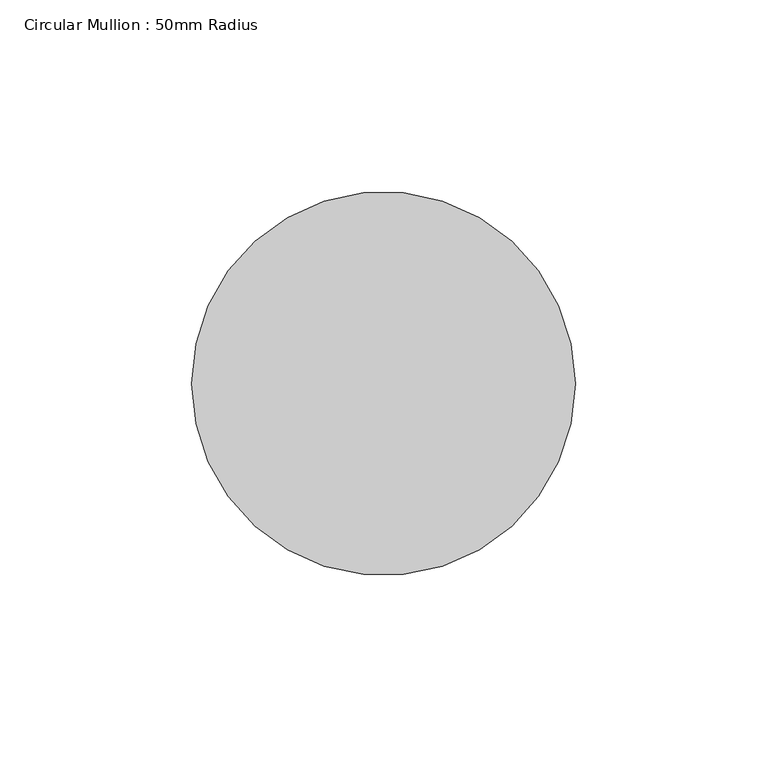
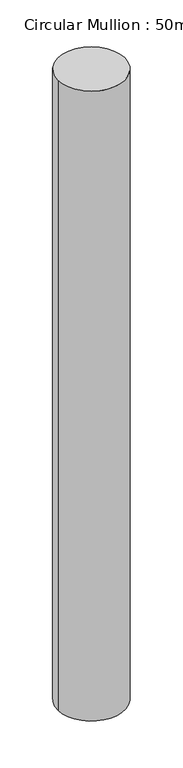
"""IFC4 building model written with IfcOpenShell, lengths in millimetres: member geometry, Circular Mullion : 50mm Radius."""

import ifcopenshell
import ifcopenshell.guid

model = None  # the IFC model being written
_history = None  # IfcOwnerHistory: only IFC2X3 demands one
_inside = {}  # id of a spatial element -> (the spatial element, [elements in it])
_under = {}  # id of a project, library or spatial element -> (it, [spatial elements below it])
_declared = {}  # id of a project -> (the project, [libraries it declares])
_typed = {}  # id of a type object -> (the type object, [elements of that type])
_made_of = {}  # id of a material, layer set ... -> (it, [elements and type objects made of it])


def new_model(schema):
    """Start an empty IFC model of exactly this schema.

    Asked for "IFC4X3", IfcOpenShell would pick the latest addendum, in which some entities
    have other attributes; the version numbers below select the first issue.
    IFC2X3 requires an IfcOwnerHistory on every rooted entity: one is made here for all.
    """
    global model, _history
    if schema == "IFC4X3":
        model = ifcopenshell.file(schema_version=(4, 3, 0, 0))
    else:
        model = ifcopenshell.file(schema=schema)
    _inside.clear()
    _under.clear()
    _declared.clear()
    _typed.clear()
    _made_of.clear()
    _history = None
    if model.schema == "IFC2X3":
        org = make("IfcOrganization", Name="unknown")
        user = make(
            "IfcPersonAndOrganization",
            ThePerson=make("IfcPerson", FamilyName="unknown"),
            TheOrganization=org,
        )
        app = make(
            "IfcApplication",
            ApplicationDeveloper=org,
            Version="unknown",
            ApplicationFullName="unknown",
            ApplicationIdentifier="unknown",
        )
        _history = make(
            "IfcOwnerHistory",
            OwningUser=user,
            OwningApplication=app,
            ChangeAction="ADDED",
            CreationDate=0,
        )
    return model


def make(cls, **values):
    """One entity of the class cls with the attributes given. An attribute that is None is left unset."""
    return model.create_entity(
        cls, **{name: value for name, value in values.items() if value is not None}
    )


def rooted(cls, **values):
    """An entity with a GlobalId (a new one), such as an element, a storey or a relation."""
    return make(cls, GlobalId=ifcopenshell.guid.new(), OwnerHistory=_history, **values)


def si_unit(unit_type, name, prefix=None):
    """IfcSIUnit, for example si_unit("LENGTHUNIT", "METRE", prefix="MILLI")."""
    return make("IfcSIUnit", UnitType=unit_type, Prefix=prefix, Name=name)


def assignment(units):
    """IfcUnitAssignment: the units of a project."""
    return None if units is None else make("IfcUnitAssignment", Units=units)


def point(xyz):
    """IfcCartesianPoint."""
    return None if xyz is None else make("IfcCartesianPoint", Coordinates=xyz)


def direction(xyz):
    """IfcDirection."""
    return None if xyz is None else make("IfcDirection", DirectionRatios=xyz)


def frame(location, z_axis=None, x_axis=None):
    """IfcAxis2Placement3D, a coordinate frame: its origin and axes. An axis left out is left unset."""
    return make(
        "IfcAxis2Placement3D",
        Location=point(location),
        Axis=direction(z_axis),
        RefDirection=direction(x_axis),
    )


def frame_2d(location, x_axis=None):
    """IfcAxis2Placement2D, a coordinate frame in the plane: its origin and x axis."""
    return make(
        "IfcAxis2Placement2D", Location=point(location), RefDirection=direction(x_axis)
    )


def origin():
    """The frame at (0, 0, 0) with its axes left unset."""
    return frame((0.0, 0.0, 0.0))


def origin_2d():
    """The frame at (0, 0) in the plane with its x axis left unset."""
    return frame_2d((0.0, 0.0))


def place(relative_to, where):
    """IfcLocalPlacement: puts the frame where relative to a parent placement (None: the world)."""
    return make(
        "IfcLocalPlacement", PlacementRelTo=relative_to, RelativePlacement=where
    )


def context(
    kind, dimensions, precision=None, world=None, true_north=None, identifier=None
):
    """IfcGeometricRepresentationContext, for example the 3D "Model" context."""
    return make(
        "IfcGeometricRepresentationContext",
        ContextIdentifier=identifier,
        ContextType=kind,
        CoordinateSpaceDimension=dimensions,
        Precision=precision,
        WorldCoordinateSystem=world,
        TrueNorth=true_north,
    )


def project(units=None, contexts=None):
    """IfcProject with its units and contexts."""
    return rooted(
        "IfcProject",
        Name="project",
        RepresentationContexts=contexts,
        UnitsInContext=assignment(units),
    )


def spatial(cls, under=None, at=None, **own):
    """A site, building, storey or space (cls), placed at a placement, below another one or the project."""
    s = rooted(cls, ObjectPlacement=at, **own)
    if under is not None:
        _under.setdefault(under.id(), (under, []))[1].append(s)
    return s


def circle_curve(where, radius):
    """IfcCircle in the frame where."""
    return make("IfcCircle", Position=where, Radius=radius)


def trimmed(basis, trim1, trim2, sense, master):
    """IfcTrimmedCurve: the piece of a basis curve between two trims."""
    return make(
        "IfcTrimmedCurve",
        BasisCurve=basis,
        Trim1=trim1,
        Trim2=trim2,
        SenseAgreement=sense,
        MasterRepresentation=master,
    )


def segment(curve, same_sense, transition):
    """IfcCompositeCurveSegment."""
    return make(
        "IfcCompositeCurveSegment",
        Transition=transition,
        SameSense=same_sense,
        ParentCurve=curve,
    )


def composite_curve(segments, self_intersect=None):
    """IfcCompositeCurve: segments joined end to end."""
    return make("IfcCompositeCurve", Segments=segments, SelfIntersect=self_intersect)


def outline(outer, holes=None, kind="AREA"):
    """IfcArbitraryClosedProfileDef: a profile drawn as a closed curve; with holes, ...WithVoids."""
    if holes is None:
        return make("IfcArbitraryClosedProfileDef", ProfileType=kind, OuterCurve=outer)
    return make(
        "IfcArbitraryProfileDefWithVoids",
        ProfileType=kind,
        OuterCurve=outer,
        InnerCurves=holes,
    )


def extrude(swept, where, along, depth):
    """IfcExtrudedAreaSolid: the profile swept, set in the frame where, extruded along a direction by depth."""
    return make(
        "IfcExtrudedAreaSolid",
        SweptArea=swept,
        Position=where,
        ExtrudedDirection=direction(along),
        Depth=depth,
    )


def shape(context_of_items, identifier, shape_type, items):
    """IfcShapeRepresentation: the items that make up one representation, for example the "Body"."""
    return make(
        "IfcShapeRepresentation",
        ContextOfItems=context_of_items,
        RepresentationIdentifier=identifier,
        RepresentationType=shape_type,
        Items=items,
    )


def source(mapping_origin, context_of_items, identifier, shape_type, items):
    """IfcRepresentationMap: a shape defined once, which mapped items show again and again."""
    return make(
        "IfcRepresentationMap",
        MappingOrigin=mapping_origin,
        MappedRepresentation=shape(context_of_items, identifier, shape_type, items),
    )


def transform(
    local_origin,
    x_axis=None,
    y_axis=None,
    z_axis=None,
    scale=None,
    scale2=None,
    scale3=None,
    uniform=True,
):
    """IfcCartesianTransformationOperator3D, or its non-uniform kind. x_axis, y_axis, z_axis: its Axis1, 2, 3."""
    if uniform:
        return make(
            "IfcCartesianTransformationOperator3D",
            Axis1=direction(x_axis),
            Axis2=direction(y_axis),
            LocalOrigin=point(local_origin),
            Scale=scale,
            Axis3=direction(z_axis),
        )
    return make(
        "IfcCartesianTransformationOperator3DnonUniform",
        Axis1=direction(x_axis),
        Axis2=direction(y_axis),
        LocalOrigin=point(local_origin),
        Scale=scale,
        Axis3=direction(z_axis),
        Scale2=scale2,
        Scale3=scale3,
    )


def mapped(mapping_source, mapping_target):
    """IfcMappedItem: shows the shape of a source again, moved by a transform."""
    return make(
        "IfcMappedItem", MappingSource=mapping_source, MappingTarget=mapping_target
    )


def made_of(thing, what):
    """Note that an element or type object is made of a material, layer set ...; save() writes the relation."""
    if what is not None:
        _made_of.setdefault(what.id(), (what, []))[1].append(thing)
    return thing


def element(
    cls,
    number,
    at=None,
    inside=None,
    cuts=None,
    type_object=None,
    material=None,
    context=None,
    identifier="Body",
    shape_type=None,
    held_by="IfcProductDefinitionShape",
    body=None,
    shapes=None,
    **own,
):
    """One element of the class cls, such as IfcWall. Its Tag is "e" and its number.

    at: its placement. inside: the storey or other place that contains it. cuts: it is an
    opening in that element (IfcRelVoidsElement). A single representation is given by context,
    identifier, shape_type and body (its items); several are given by shapes. held_by: the class
    of the entity that holds the representations. save() writes the other relations.
    """
    e = rooted(cls, Tag="e%d" % number, ObjectPlacement=at, **own)
    if body is not None:
        shapes = [shape(context, identifier, shape_type, body)]
    if shapes is not None:
        e.Representation = make(held_by, Representations=shapes)
    if inside is not None:
        _inside.setdefault(inside.id(), (inside, []))[1].append(e)
    if cuts is not None:
        rooted(
            "IfcRelVoidsElement", RelatingBuildingElement=cuts, RelatedOpeningElement=e
        )
    if type_object is not None:
        _typed.setdefault(type_object.id(), (type_object, []))[1].append(e)
    return made_of(e, material)


def aggregate(whole, parts):
    """IfcRelAggregates: a whole, such as a stair, and the parts it consists of."""
    return rooted("IfcRelAggregates", RelatingObject=whole, RelatedObjects=parts)


def save(model, path):
    """Write the relations noted so far, then the file.

    IfcRelAggregates (storeys below a building ...), IfcRelContainedInSpatialStructure (elements
    in a storey), IfcRelDefinesByType, IfcRelAssociatesMaterial and IfcRelDeclares: one each for
    every whole, place, type object, material and project.
    """
    for whole, parts in _under.values():
        aggregate(whole, parts)
    for where, things in _inside.values():
        rooted(
            "IfcRelContainedInSpatialStructure",
            RelatedElements=things,
            RelatingStructure=where,
        )
    for kind, things in _typed.values():
        rooted("IfcRelDefinesByType", RelatedObjects=things, RelatingType=kind)
    for what, things in _made_of.values():
        rooted("IfcRelAssociatesMaterial", RelatedObjects=things, RelatingMaterial=what)
    for by, libraries in _declared.values():
        rooted("IfcRelDeclares", RelatingContext=by, RelatedDefinitions=libraries)
    model.write(path)


def circular_mullion_50mm_radius_7177ed17(model_context):
    return source(origin(), model_context, "Body", "SweptSolid", [
        extrude(outline(composite_curve([segment(trimmed(circle_curve(origin_2d(), 50.0), [point((50.0, 0.0))], [point((-50.0, 0.0))], False, "CARTESIAN"), True, "CONTINUOUS"), segment(trimmed(circle_curve(origin_2d(), 50.0), [point((-50.0, 0.0))], [point((50.0, 0.0))], False, "CARTESIAN"), True, "CONTINUOUS")], self_intersect=False)), frame((0.0, 0.0, -993.4713594), z_axis=(0.0, 0.0, 1.0), x_axis=(1.0, 0.0, 0.0)), (0.0, 0.0, 1.0), 993.4713594),
    ])


if __name__ == "__main__":
    model = new_model("IFC4")
    model_context = context("Model", 3, world=origin())
    ifc_project = project(units=[si_unit("LENGTHUNIT", "METRE", prefix="MILLI")], contexts=[model_context])
    site = spatial("IfcSite", under=ifc_project)
    building = spatial("IfcBuilding", under=site)
    placement = place(None, origin())
    circular_mullion_50mm_radius_shape = circular_mullion_50mm_radius_7177ed17(model_context)
    element("IfcMember", 1, ObjectType="Circular Mullion : 50mm Radius", at=placement, inside=building, context=model_context, shape_type="MappedRepresentation", body=[
        mapped(circular_mullion_50mm_radius_shape, transform((0.0, 0.0, 0.0), x_axis=(1.0, 0.0, 0.0), y_axis=(0.0, 1.0, 0.0), z_axis=(0.0, 0.0, 1.0))),
    ])
    save(model, "model.ifc")

# Revit data of these elements
# Type "Circular Mullion : 50mm Radius"
#   built-in parameter 1007350 = 0.164042 (stored number, unit not read)
# Element 1 (IfcMember, "Circular Mullion : 50mm Radius")
#   Materials on its faces: "Aluminium"
# Materials
#   "Aluminium": class "Metal", colour RGB 247 247 247, transparency 0, Description = "Aluminium 6061", Cost = 0
